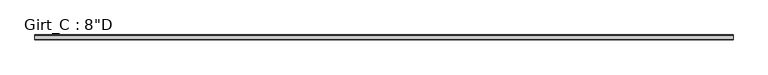
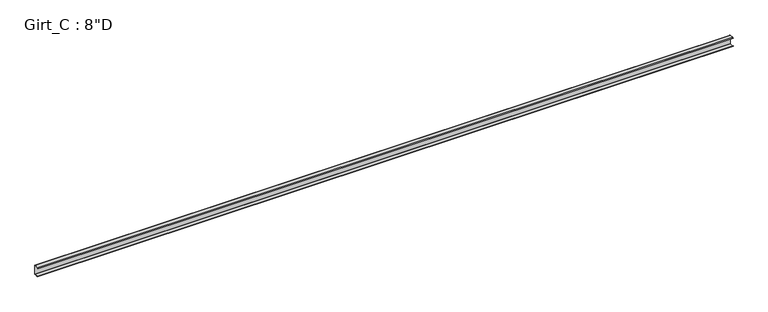
"""IFC4 building model written with IfcOpenShell, lengths in millimetres: beam geometry."""

import ifcopenshell
import ifcopenshell.guid

model = None  # the IFC model being written
_history = None  # IfcOwnerHistory: only IFC2X3 demands one
_inside = {}  # id of a spatial element -> (the spatial element, [elements in it])
_under = {}  # id of a project, library or spatial element -> (it, [spatial elements below it])
_declared = {}  # id of a project -> (the project, [libraries it declares])
_typed = {}  # id of a type object -> (the type object, [elements of that type])
_made_of = {}  # id of a material, layer set ... -> (it, [elements and type objects made of it])


def new_model(schema):
    """Start an empty IFC model of exactly this schema.

    Asked for "IFC4X3", IfcOpenShell would pick the latest addendum, in which some entities
    have other attributes; the version numbers below select the first issue.
    IFC2X3 requires an IfcOwnerHistory on every rooted entity: one is made here for all.
    """
    global model, _history
    if schema == "IFC4X3":
        model = ifcopenshell.file(schema_version=(4, 3, 0, 0))
    else:
        model = ifcopenshell.file(schema=schema)
    _inside.clear()
    _under.clear()
    _declared.clear()
    _typed.clear()
    _made_of.clear()
    _history = None
    if model.schema == "IFC2X3":
        org = make("IfcOrganization", Name="unknown")
        user = make(
            "IfcPersonAndOrganization",
            ThePerson=make("IfcPerson", FamilyName="unknown"),
            TheOrganization=org,
        )
        app = make(
            "IfcApplication",
            ApplicationDeveloper=org,
            Version="unknown",
            ApplicationFullName="unknown",
            ApplicationIdentifier="unknown",
        )
        _history = make(
            "IfcOwnerHistory",
            OwningUser=user,
            OwningApplication=app,
            ChangeAction="ADDED",
            CreationDate=0,
        )
    return model


def make(cls, **values):
    """One entity of the class cls with the attributes given. An attribute that is None is left unset."""
    return model.create_entity(
        cls, **{name: value for name, value in values.items() if value is not None}
    )


def rooted(cls, **values):
    """An entity with a GlobalId (a new one), such as an element, a storey or a relation."""
    return make(cls, GlobalId=ifcopenshell.guid.new(), OwnerHistory=_history, **values)


def si_unit(unit_type, name, prefix=None):
    """IfcSIUnit, for example si_unit("LENGTHUNIT", "METRE", prefix="MILLI")."""
    return make("IfcSIUnit", UnitType=unit_type, Prefix=prefix, Name=name)


def assignment(units):
    """IfcUnitAssignment: the units of a project."""
    return None if units is None else make("IfcUnitAssignment", Units=units)


def point(xyz):
    """IfcCartesianPoint."""
    return None if xyz is None else make("IfcCartesianPoint", Coordinates=xyz)


def direction(xyz):
    """IfcDirection."""
    return None if xyz is None else make("IfcDirection", DirectionRatios=xyz)


def frame(location, z_axis=None, x_axis=None):
    """IfcAxis2Placement3D, a coordinate frame: its origin and axes. An axis left out is left unset."""
    return make(
        "IfcAxis2Placement3D",
        Location=point(location),
        Axis=direction(z_axis),
        RefDirection=direction(x_axis),
    )


def frame_2d(location, x_axis=None):
    """IfcAxis2Placement2D, a coordinate frame in the plane: its origin and x axis."""
    return make(
        "IfcAxis2Placement2D", Location=point(location), RefDirection=direction(x_axis)
    )


def origin():
    """The frame at (0, 0, 0) with its axes left unset."""
    return frame((0.0, 0.0, 0.0))


def place(relative_to, where):
    """IfcLocalPlacement: puts the frame where relative to a parent placement (None: the world)."""
    return make(
        "IfcLocalPlacement", PlacementRelTo=relative_to, RelativePlacement=where
    )


def context(
    kind, dimensions, precision=None, world=None, true_north=None, identifier=None
):
    """IfcGeometricRepresentationContext, for example the 3D "Model" context."""
    return make(
        "IfcGeometricRepresentationContext",
        ContextIdentifier=identifier,
        ContextType=kind,
        CoordinateSpaceDimension=dimensions,
        Precision=precision,
        WorldCoordinateSystem=world,
        TrueNorth=true_north,
    )


def project(units=None, contexts=None):
    """IfcProject with its units and contexts."""
    return rooted(
        "IfcProject",
        Name="project",
        RepresentationContexts=contexts,
        UnitsInContext=assignment(units),
    )


def spatial(cls, under=None, at=None, **own):
    """A site, building, storey or space (cls), placed at a placement, below another one or the project."""
    s = rooted(cls, ObjectPlacement=at, **own)
    if under is not None:
        _under.setdefault(under.id(), (under, []))[1].append(s)
    return s


def polyline(points):
    """IfcPolyline through the points."""
    return make("IfcPolyline", Points=[point(p) for p in points])


def circle_curve(where, radius):
    """IfcCircle in the frame where."""
    return make("IfcCircle", Position=where, Radius=radius)


def trimmed(basis, trim1, trim2, sense, master):
    """IfcTrimmedCurve: the piece of a basis curve between two trims."""
    return make(
        "IfcTrimmedCurve",
        BasisCurve=basis,
        Trim1=trim1,
        Trim2=trim2,
        SenseAgreement=sense,
        MasterRepresentation=master,
    )


def segment(curve, same_sense, transition):
    """IfcCompositeCurveSegment."""
    return make(
        "IfcCompositeCurveSegment",
        Transition=transition,
        SameSense=same_sense,
        ParentCurve=curve,
    )


def composite_curve(segments, self_intersect=None):
    """IfcCompositeCurve: segments joined end to end."""
    return make("IfcCompositeCurve", Segments=segments, SelfIntersect=self_intersect)


def outline(outer, holes=None, kind="AREA"):
    """IfcArbitraryClosedProfileDef: a profile drawn as a closed curve; with holes, ...WithVoids."""
    if holes is None:
        return make("IfcArbitraryClosedProfileDef", ProfileType=kind, OuterCurve=outer)
    return make(
        "IfcArbitraryProfileDefWithVoids",
        ProfileType=kind,
        OuterCurve=outer,
        InnerCurves=holes,
    )


def extrude(swept, where, along, depth):
    """IfcExtrudedAreaSolid: the profile swept, set in the frame where, extruded along a direction by depth."""
    return make(
        "IfcExtrudedAreaSolid",
        SweptArea=swept,
        Position=where,
        ExtrudedDirection=direction(along),
        Depth=depth,
    )


def shape(context_of_items, identifier, shape_type, items):
    """IfcShapeRepresentation: the items that make up one representation, for example the "Body"."""
    return make(
        "IfcShapeRepresentation",
        ContextOfItems=context_of_items,
        RepresentationIdentifier=identifier,
        RepresentationType=shape_type,
        Items=items,
    )


def source(mapping_origin, context_of_items, identifier, shape_type, items):
    """IfcRepresentationMap: a shape defined once, which mapped items show again and again."""
    return make(
        "IfcRepresentationMap",
        MappingOrigin=mapping_origin,
        MappedRepresentation=shape(context_of_items, identifier, shape_type, items),
    )


def transform(
    local_origin,
    x_axis=None,
    y_axis=None,
    z_axis=None,
    scale=None,
    scale2=None,
    scale3=None,
    uniform=True,
):
    """IfcCartesianTransformationOperator3D, or its non-uniform kind. x_axis, y_axis, z_axis: its Axis1, 2, 3."""
    if uniform:
        return make(
            "IfcCartesianTransformationOperator3D",
            Axis1=direction(x_axis),
            Axis2=direction(y_axis),
            LocalOrigin=point(local_origin),
            Scale=scale,
            Axis3=direction(z_axis),
        )
    return make(
        "IfcCartesianTransformationOperator3DnonUniform",
        Axis1=direction(x_axis),
        Axis2=direction(y_axis),
        LocalOrigin=point(local_origin),
        Scale=scale,
        Axis3=direction(z_axis),
        Scale2=scale2,
        Scale3=scale3,
    )


def mapped(mapping_source, mapping_target):
    """IfcMappedItem: shows the shape of a source again, moved by a transform."""
    return make(
        "IfcMappedItem", MappingSource=mapping_source, MappingTarget=mapping_target
    )


def made_of(thing, what):
    """Note that an element or type object is made of a material, layer set ...; save() writes the relation."""
    if what is not None:
        _made_of.setdefault(what.id(), (what, []))[1].append(thing)
    return thing


def element(
    cls,
    number,
    at=None,
    inside=None,
    cuts=None,
    type_object=None,
    material=None,
    context=None,
    identifier="Body",
    shape_type=None,
    held_by="IfcProductDefinitionShape",
    body=None,
    shapes=None,
    **own,
):
    """One element of the class cls, such as IfcWall. Its Tag is "e" and its number.

    at: its placement. inside: the storey or other place that contains it. cuts: it is an
    opening in that element (IfcRelVoidsElement). A single representation is given by context,
    identifier, shape_type and body (its items); several are given by shapes. held_by: the class
    of the entity that holds the representations. save() writes the other relations.
    """
    e = rooted(cls, Tag="e%d" % number, ObjectPlacement=at, **own)
    if body is not None:
        shapes = [shape(context, identifier, shape_type, body)]
    if shapes is not None:
        e.Representation = make(held_by, Representations=shapes)
    if inside is not None:
        _inside.setdefault(inside.id(), (inside, []))[1].append(e)
    if cuts is not None:
        rooted(
            "IfcRelVoidsElement", RelatingBuildingElement=cuts, RelatedOpeningElement=e
        )
    if type_object is not None:
        _typed.setdefault(type_object.id(), (type_object, []))[1].append(e)
    return made_of(e, material)


def aggregate(whole, parts):
    """IfcRelAggregates: a whole, such as a stair, and the parts it consists of."""
    return rooted("IfcRelAggregates", RelatingObject=whole, RelatedObjects=parts)


def save(model, path):
    """Write the relations noted so far, then the file.

    IfcRelAggregates (storeys below a building ...), IfcRelContainedInSpatialStructure (elements
    in a storey), IfcRelDefinesByType, IfcRelAssociatesMaterial and IfcRelDeclares: one each for
    every whole, place, type object, material and project.
    """
    for whole, parts in _under.values():
        aggregate(whole, parts)
    for where, things in _inside.values():
        rooted(
            "IfcRelContainedInSpatialStructure",
            RelatedElements=things,
            RelatingStructure=where,
        )
    for kind, things in _typed.values():
        rooted("IfcRelDefinesByType", RelatedObjects=things, RelatingType=kind)
    for what, things in _made_of.values():
        rooted("IfcRelAssociatesMaterial", RelatedObjects=things, RelatingMaterial=what)
    for by, libraries in _declared.values():
        rooted("IfcRelDeclares", RelatingContext=by, RelatedDefinitions=libraries)
    model.write(path)


def beam_dc045d9c(model_context):
    return source(origin(), model_context, "Body", "SweptSolid", [
        extrude(outline(composite_curve([segment(polyline([(-87.5109375, 101.6), (-3.3734375, 101.6)]), True, "CONTINUOUS"), segment(trimmed(circle_curve(frame_2d((-3.3734375, 96.8375)), 4.7625), [point((-3.3734375, 101.6))], [point((1.3890625, 96.8375))], False, "CARTESIAN"), True, "CONTINUOUS"), segment(polyline([(1.3890625, 96.8375), (1.3890625, -96.8375)]), True, "CONTINUOUS"), segment(trimmed(circle_curve(frame_2d((-3.3734375, -96.8375)), 4.7625), [point((1.3890625, -96.8375))], [point((-3.3734375, -101.6))], False, "CARTESIAN"), True, "CONTINUOUS"), segment(polyline([(-3.3734375, -101.6), (-87.5109375, -101.6), (-99.7792647, -86.979177), (-97.6510975, -85.1934327), (-86.2154765, -98.821875), (-3.2694106, -98.821875)]), True, "CONTINUOUS"), segment(trimmed(circle_curve(frame_2d((-3.3748024, -96.8389339)), 1.9857399), [point((-3.2694106, -98.821875))], [point((-1.3890625, -96.8389339))], True, "CARTESIAN"), True, "CONTINUOUS"), segment(polyline([(-1.3890625, -96.8389339), (-1.3890625, 96.8381931)]), True, "CONTINUOUS"), segment(trimmed(circle_curve(frame_2d((-3.3741066, 96.8381931)), 1.9850441), [point((-1.3890625, 96.8381931))], [point((-3.3005807, 98.821875))], True, "CARTESIAN"), True, "CONTINUOUS"), segment(polyline([(-3.3005807, 98.821875), (-86.2154765, 98.821875), (-97.6278742, 85.221109), (-99.7560415, 87.0068534), (-87.5109375, 101.6)]), True, "CONTINUOUS")], self_intersect=False)), frame((-7471.171875, 0.0, 0.0), z_axis=(1.0, 0.0, 0.0), x_axis=(0.0, 1.0, 0.0)), (0.0, 0.0, 1.0), 14789.15),
    ])


if __name__ == "__main__":
    model = new_model("IFC4")
    model_context = context("Model", 3, world=origin())
    ifc_project = project(units=[si_unit("LENGTHUNIT", "METRE", prefix="MILLI")], contexts=[model_context])
    site = spatial("IfcSite", under=ifc_project)
    building = spatial("IfcBuilding", under=site)
    placement = place(None, origin())
    beam_shape = beam_dc045d9c(model_context)
    element("IfcBeam", 1, ObjectType="Girt_C : 8\"D", at=placement, inside=building, context=model_context, shape_type="MappedRepresentation", body=[
        mapped(beam_shape, transform((0.0, 0.0, 0.0), x_axis=(1.0, 0.0, 0.0), y_axis=(0.0, 1.0, 0.0), z_axis=(0.0, 0.0, 1.0))),
    ])
    save(model, "model.ifc")

# Revit data of these elements
# Type "Girt_C : 8\"D"
#   half leg = 0' - 1 3/4"
#   Web_Thickness = 0' - 0 7/64"
#   Length [instance default] = 10' - 0"
#   Leg_1 = 0' - 3 1/2"
#   Height = 0' - 8"
#   Structural Material [instance default] = none
# Element 1 (IfcBeam, "Girt_C : 8\"D")
#   Structural Material = GALVANIZED 'CEE' SECTION (8.0x3.5C - SEE STRUCT. DWGS)
#   Materials on its faces: "GALVANIZED 'CEE' SECTION (8.0x3.5C - SEE STRUCT. DWGS)"
# Materials
#   "GALVANIZED 'CEE' SECTION (8.0x3.5C - SEE STRUCT. DWGS)": class "Metal", colour RGB 137 146 153, transparency 0, Description = "Steel, mill finish", Cost = 0
